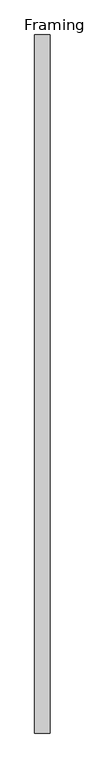
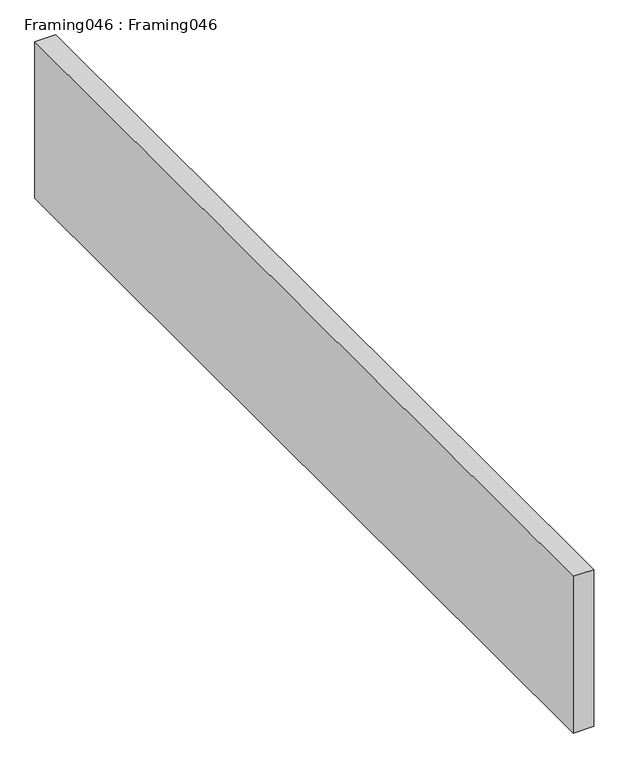
"""IFC4 building model written with IfcOpenShell, lengths in millimetres: proxy geometry, Framing046 : Framing046."""

from ifc_helpers import new_model, si_unit, frame, origin, place, context, project, spatial, polyline, outline, extrude, source, transform, mapped, element, save


def framing046_framing046_3661c0d5(model_context):
    return source(origin(), model_context, "Body", "SweptSolid", [
        extrude(outline(polyline([(-4313.3493999, 7982.1531721), (-4357.7993999, 7982.1531721), (-4357.7993999, 9982.1531721), (-4313.3493999, 9982.1531721), (-4313.3493999, 7982.1531721)])), frame((0.0, 0.0, 43056.5101822), z_axis=(0.0, 0.0, 1.0), x_axis=(1.0, 0.0, 0.0)), (0.0, 0.0, 1.0), 355.2981173),
    ])


if __name__ == "__main__":
    model = new_model("IFC4")
    model_context = context("Model", 3, world=origin())
    ifc_project = project(units=[si_unit("LENGTHUNIT", "METRE", prefix="MILLI")], contexts=[model_context])
    site = spatial("IfcSite", under=ifc_project)
    building = spatial("IfcBuilding", under=site)
    placement = place(None, origin())
    framing046_framing046_shape = framing046_framing046_3661c0d5(model_context)
    element("IfcBuildingElementProxy", 1, Name="Framing046 : Framing046", ObjectType="Framing046 : Framing046", at=placement, inside=building, context=model_context, shape_type="MappedRepresentation", body=[
        mapped(framing046_framing046_shape, transform((0.0, 0.0, 0.0), x_axis=(1.0, 0.0, 0.0), y_axis=(0.0, 1.0, 0.0), z_axis=(0.0, 0.0, 1.0))),
    ])
    save(model, "model.ifc")

# Revit data of these elements
# Type "Framing046 : Framing046"
#   NameOverride = "Framing046"
# Element 1 (IfcBuildingElementProxy, "Framing046 : Framing046")
#   Materials on its faces: "WOOD FRAMING (SEE STRUCT DWGS)"
# Materials
#   "WOOD FRAMING (SEE STRUCT DWGS)": class "Unassigned", colour RGB 224 188 168, transparency 0, Cost = 0
